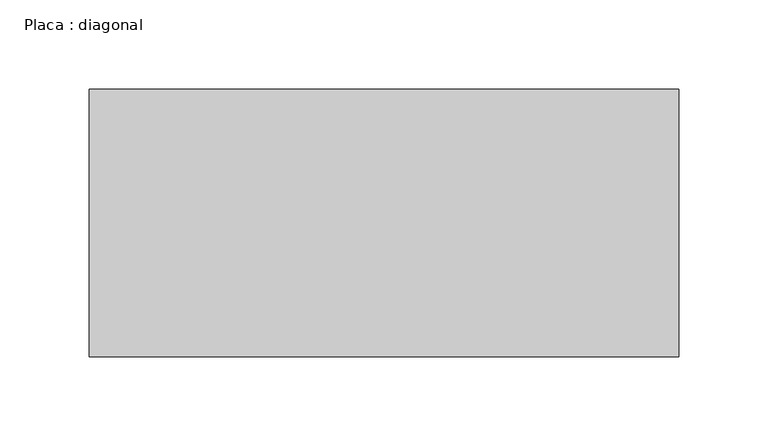
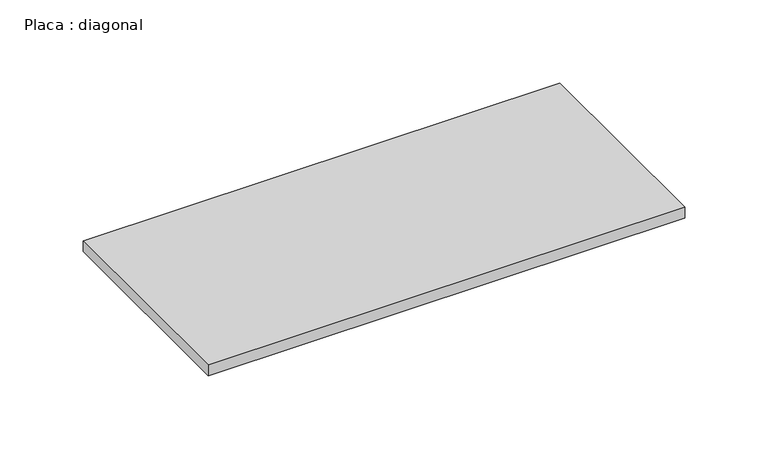
"""IFC4 building model written with IfcOpenShell, lengths in millimetres: beam geometry, Placa : diagonal."""

import ifcopenshell
import ifcopenshell.guid

model = None  # the IFC model being written
_history = None  # IfcOwnerHistory: only IFC2X3 demands one
_inside = {}  # id of a spatial element -> (the spatial element, [elements in it])
_under = {}  # id of a project, library or spatial element -> (it, [spatial elements below it])
_declared = {}  # id of a project -> (the project, [libraries it declares])
_typed = {}  # id of a type object -> (the type object, [elements of that type])
_made_of = {}  # id of a material, layer set ... -> (it, [elements and type objects made of it])


def new_model(schema):
    """Start an empty IFC model of exactly this schema.

    Asked for "IFC4X3", IfcOpenShell would pick the latest addendum, in which some entities
    have other attributes; the version numbers below select the first issue.
    IFC2X3 requires an IfcOwnerHistory on every rooted entity: one is made here for all.
    """
    global model, _history
    if schema == "IFC4X3":
        model = ifcopenshell.file(schema_version=(4, 3, 0, 0))
    else:
        model = ifcopenshell.file(schema=schema)
    _inside.clear()
    _under.clear()
    _declared.clear()
    _typed.clear()
    _made_of.clear()
    _history = None
    if model.schema == "IFC2X3":
        org = make("IfcOrganization", Name="unknown")
        user = make(
            "IfcPersonAndOrganization",
            ThePerson=make("IfcPerson", FamilyName="unknown"),
            TheOrganization=org,
        )
        app = make(
            "IfcApplication",
            ApplicationDeveloper=org,
            Version="unknown",
            ApplicationFullName="unknown",
            ApplicationIdentifier="unknown",
        )
        _history = make(
            "IfcOwnerHistory",
            OwningUser=user,
            OwningApplication=app,
            ChangeAction="ADDED",
            CreationDate=0,
        )
    return model


def make(cls, **values):
    """One entity of the class cls with the attributes given. An attribute that is None is left unset."""
    return model.create_entity(
        cls, **{name: value for name, value in values.items() if value is not None}
    )


def rooted(cls, **values):
    """An entity with a GlobalId (a new one), such as an element, a storey or a relation."""
    return make(cls, GlobalId=ifcopenshell.guid.new(), OwnerHistory=_history, **values)


def si_unit(unit_type, name, prefix=None):
    """IfcSIUnit, for example si_unit("LENGTHUNIT", "METRE", prefix="MILLI")."""
    return make("IfcSIUnit", UnitType=unit_type, Prefix=prefix, Name=name)


def assignment(units):
    """IfcUnitAssignment: the units of a project."""
    return None if units is None else make("IfcUnitAssignment", Units=units)


def point(xyz):
    """IfcCartesianPoint."""
    return None if xyz is None else make("IfcCartesianPoint", Coordinates=xyz)


def direction(xyz):
    """IfcDirection."""
    return None if xyz is None else make("IfcDirection", DirectionRatios=xyz)


def frame(location, z_axis=None, x_axis=None):
    """IfcAxis2Placement3D, a coordinate frame: its origin and axes. An axis left out is left unset."""
    return make(
        "IfcAxis2Placement3D",
        Location=point(location),
        Axis=direction(z_axis),
        RefDirection=direction(x_axis),
    )


def origin():
    """The frame at (0, 0, 0) with its axes left unset."""
    return frame((0.0, 0.0, 0.0))


def place(relative_to, where):
    """IfcLocalPlacement: puts the frame where relative to a parent placement (None: the world)."""
    return make(
        "IfcLocalPlacement", PlacementRelTo=relative_to, RelativePlacement=where
    )


def context(
    kind, dimensions, precision=None, world=None, true_north=None, identifier=None
):
    """IfcGeometricRepresentationContext, for example the 3D "Model" context."""
    return make(
        "IfcGeometricRepresentationContext",
        ContextIdentifier=identifier,
        ContextType=kind,
        CoordinateSpaceDimension=dimensions,
        Precision=precision,
        WorldCoordinateSystem=world,
        TrueNorth=true_north,
    )


def project(units=None, contexts=None):
    """IfcProject with its units and contexts."""
    return rooted(
        "IfcProject",
        Name="project",
        RepresentationContexts=contexts,
        UnitsInContext=assignment(units),
    )


def spatial(cls, under=None, at=None, **own):
    """A site, building, storey or space (cls), placed at a placement, below another one or the project."""
    s = rooted(cls, ObjectPlacement=at, **own)
    if under is not None:
        _under.setdefault(under.id(), (under, []))[1].append(s)
    return s


def polyline(points):
    """IfcPolyline through the points."""
    return make("IfcPolyline", Points=[point(p) for p in points])


def outline(outer, holes=None, kind="AREA"):
    """IfcArbitraryClosedProfileDef: a profile drawn as a closed curve; with holes, ...WithVoids."""
    if holes is None:
        return make("IfcArbitraryClosedProfileDef", ProfileType=kind, OuterCurve=outer)
    return make(
        "IfcArbitraryProfileDefWithVoids",
        ProfileType=kind,
        OuterCurve=outer,
        InnerCurves=holes,
    )


def extrude(swept, where, along, depth):
    """IfcExtrudedAreaSolid: the profile swept, set in the frame where, extruded along a direction by depth."""
    return make(
        "IfcExtrudedAreaSolid",
        SweptArea=swept,
        Position=where,
        ExtrudedDirection=direction(along),
        Depth=depth,
    )


def shape(context_of_items, identifier, shape_type, items):
    """IfcShapeRepresentation: the items that make up one representation, for example the "Body"."""
    return make(
        "IfcShapeRepresentation",
        ContextOfItems=context_of_items,
        RepresentationIdentifier=identifier,
        RepresentationType=shape_type,
        Items=items,
    )


def source(mapping_origin, context_of_items, identifier, shape_type, items):
    """IfcRepresentationMap: a shape defined once, which mapped items show again and again."""
    return make(
        "IfcRepresentationMap",
        MappingOrigin=mapping_origin,
        MappedRepresentation=shape(context_of_items, identifier, shape_type, items),
    )


def transform(
    local_origin,
    x_axis=None,
    y_axis=None,
    z_axis=None,
    scale=None,
    scale2=None,
    scale3=None,
    uniform=True,
):
    """IfcCartesianTransformationOperator3D, or its non-uniform kind. x_axis, y_axis, z_axis: its Axis1, 2, 3."""
    if uniform:
        return make(
            "IfcCartesianTransformationOperator3D",
            Axis1=direction(x_axis),
            Axis2=direction(y_axis),
            LocalOrigin=point(local_origin),
            Scale=scale,
            Axis3=direction(z_axis),
        )
    return make(
        "IfcCartesianTransformationOperator3DnonUniform",
        Axis1=direction(x_axis),
        Axis2=direction(y_axis),
        LocalOrigin=point(local_origin),
        Scale=scale,
        Axis3=direction(z_axis),
        Scale2=scale2,
        Scale3=scale3,
    )


def mapped(mapping_source, mapping_target):
    """IfcMappedItem: shows the shape of a source again, moved by a transform."""
    return make(
        "IfcMappedItem", MappingSource=mapping_source, MappingTarget=mapping_target
    )


def made_of(thing, what):
    """Note that an element or type object is made of a material, layer set ...; save() writes the relation."""
    if what is not None:
        _made_of.setdefault(what.id(), (what, []))[1].append(thing)
    return thing


def element(
    cls,
    number,
    at=None,
    inside=None,
    cuts=None,
    type_object=None,
    material=None,
    context=None,
    identifier="Body",
    shape_type=None,
    held_by="IfcProductDefinitionShape",
    body=None,
    shapes=None,
    **own,
):
    """One element of the class cls, such as IfcWall. Its Tag is "e" and its number.

    at: its placement. inside: the storey or other place that contains it. cuts: it is an
    opening in that element (IfcRelVoidsElement). A single representation is given by context,
    identifier, shape_type and body (its items); several are given by shapes. held_by: the class
    of the entity that holds the representations. save() writes the other relations.
    """
    e = rooted(cls, Tag="e%d" % number, ObjectPlacement=at, **own)
    if body is not None:
        shapes = [shape(context, identifier, shape_type, body)]
    if shapes is not None:
        e.Representation = make(held_by, Representations=shapes)
    if inside is not None:
        _inside.setdefault(inside.id(), (inside, []))[1].append(e)
    if cuts is not None:
        rooted(
            "IfcRelVoidsElement", RelatingBuildingElement=cuts, RelatedOpeningElement=e
        )
    if type_object is not None:
        _typed.setdefault(type_object.id(), (type_object, []))[1].append(e)
    return made_of(e, material)


def aggregate(whole, parts):
    """IfcRelAggregates: a whole, such as a stair, and the parts it consists of."""
    return rooted("IfcRelAggregates", RelatingObject=whole, RelatedObjects=parts)


def save(model, path):
    """Write the relations noted so far, then the file.

    IfcRelAggregates (storeys below a building ...), IfcRelContainedInSpatialStructure (elements
    in a storey), IfcRelDefinesByType, IfcRelAssociatesMaterial and IfcRelDeclares: one each for
    every whole, place, type object, material and project.
    """
    for whole, parts in _under.values():
        aggregate(whole, parts)
    for where, things in _inside.values():
        rooted(
            "IfcRelContainedInSpatialStructure",
            RelatedElements=things,
            RelatingStructure=where,
        )
    for kind, things in _typed.values():
        rooted("IfcRelDefinesByType", RelatedObjects=things, RelatingType=kind)
    for what, things in _made_of.values():
        rooted("IfcRelAssociatesMaterial", RelatedObjects=things, RelatingMaterial=what)
    for by, libraries in _declared.values():
        rooted("IfcRelDeclares", RelatingContext=by, RelatedDefinitions=libraries)
    model.write(path)


def placa_diagonal_d1da0e1c(model_context):
    return source(origin(), model_context, "Body", "SweptSolid", [
        extrude(outline(polyline([(165.1705221, 75.0), (165.1705221, -75.0), (-165.4962734, -75.0), (-165.4962734, 75.0), (165.1705221, 75.0)])), frame((0.0, 0.0, -4.0), z_axis=(0.0, 0.0, 1.0), x_axis=(1.0, 0.0, 0.0)), (0.0, 0.0, 1.0), 8.0),
    ])


if __name__ == "__main__":
    model = new_model("IFC4")
    model_context = context("Model", 3, world=origin())
    ifc_project = project(units=[si_unit("LENGTHUNIT", "METRE", prefix="MILLI")], contexts=[model_context])
    site = spatial("IfcSite", under=ifc_project)
    building = spatial("IfcBuilding", under=site)
    placement = place(None, origin())
    placa_diagonal_shape = placa_diagonal_d1da0e1c(model_context)
    element("IfcBeam", 1, ObjectType="Placa : diagonal", at=placement, inside=building, context=model_context, shape_type="MappedRepresentation", body=[
        mapped(placa_diagonal_shape, transform((0.0, 0.0, 0.0), x_axis=(1.0, 0.0, 0.0), y_axis=(0.0, 1.0, 0.0), z_axis=(0.0, 0.0, 1.0))),
    ])
    save(model, "model.ifc")

# Revit data of these elements
# Type "Placa : diagonal"
#   W = 0
#   Length [instance default] = 1.50 m
#   b = 0.15 m
#   d = 0.008 m
#   A = 0 m²
#   Structural Material [instance default] = Aço, 45-345
# Element 1 (IfcBeam, "Placa : diagonal")
#   Materials on its faces: "Aço, 45-345"
# Materials
#   "Aço, 45-345": class "Metal", colour RGB 247 247 247, transparency 0, Description = "Aço 345 MPa", Cost = 0
